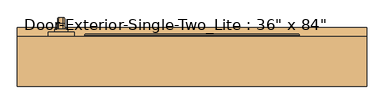
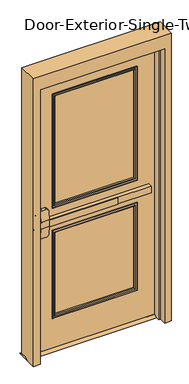
"""IFC4 building model written with IfcOpenShell, lengths in millimetres: door geometry."""

from ifc_helpers import new_model, si_unit, point, frame, frame_2d, origin, place, context, project, spatial, polyline, circle_curve, ellipse_curve, trimmed, segment, composite_curve, outline, extrude, faceted_brep, source, transform, mapped, element, save
from ifc_brep_helpers import plane_surface, cylinder_surface, revolved_surface, advanced_brep


def door_ea45fa4a(model_context):
    return source(origin(), model_context, "Body", "SolidModel", [
        extrude(outline(polyline([(61.9125, 12.7), (106.3625, 12.7), (131.7625, 0.0), (36.5125, 0.0), (61.9125, 12.7)])), frame((-508.0, 0.0, 0.0), z_axis=(1.0, 0.0, 0.0), x_axis=(0.0, 1.0, 0.0)), (0.0, 0.0, 1.0), 1016.0),
        extrude(outline(polyline([(150.2833333, 23.8125), (-349.25, 23.8125), (-349.25, 30.1625), (150.2833333, 30.1625), (150.2833333, 23.8125)])), frame((0.0, 0.0, 990.6), z_axis=(0.0, 0.0, 1.0), x_axis=(1.0, 0.0, 0.0)), (0.0, 0.0, 1.0), 50.8),
        advanced_brep(
        [(-412.75, 30.1625, 1041.4), (-412.75, 30.1625, 990.6), (-349.25, 30.1625, 990.6), (400.05, 30.1625, 990.6), (400.05, 30.1625, 1041.4), (-349.25, 30.1625, 1041.4), (400.05, 61.9125, 1041.4), (400.05, 61.9125, 990.6), (-349.25, 61.9125, 990.6), (-349.25, 61.9125, 927.1), (-368.3, 61.9125, 908.05), (-393.7, 61.9125, 908.05), (-412.75, 61.9125, 927.1), (-412.75, 61.9125, 1104.9), (-393.7, 61.9125, 1123.95), (-368.3, 61.9125, 1123.95), (-349.25, 61.9125, 1104.9), (-349.25, 61.9125, 1041.4), (-349.25, 33.3377467, 1041.4), (-412.75, 33.3377467, 1041.4), (-412.75, 38.3479269, 1104.9), (-412.75, 38.3479269, 927.1), (-412.75, 33.3377467, 990.6), (-349.25, 33.3377467, 990.6), (-349.25, 38.3479269, 927.1), (-349.25, 38.3479269, 1104.9), (-393.7, 39.850981, 1123.95), (-368.3, 39.850981, 1123.95), (-368.3, 39.850981, 908.05), (-393.7, 39.850981, 908.05)],
        [
            (0, 1),
            (1, 2),
            (2, 3),
            (3, 4),
            (4, 5),
            (5, 0),
            (6, 7),
            (7, 8),
            (8, 9),
            (9, 10, circle_curve(frame((-368.3, 61.9125, 927.1), z_axis=(0.0, 1.0, 0.0), x_axis=(1.0, 0.0, 0.0)), 19.05)),
            (10, 11),
            (11, 12, circle_curve(frame((-393.7, 61.9125, 927.1), z_axis=(0.0, 1.0, 0.0), x_axis=(1.0, 0.0, 0.0)), 19.05)),
            (12, 13),
            (13, 14, circle_curve(frame((-393.7, 61.9125, 1104.9), z_axis=(0.0, 1.0, 0.0), x_axis=(1.0, 0.0, 0.0)), 19.05)),
            (14, 15),
            (15, 16, circle_curve(frame((-368.3, 61.9125, 1104.9), z_axis=(0.0, 1.0, 0.0), x_axis=(1.0, 0.0, 0.0)), 19.05)),
            (16, 17),
            (17, 6),
            (4, 6),
            (17, 18),
            (18, 19),
            (19, 0),
            (19, 20),
            (20, 13),
            (12, 21),
            (21, 22),
            (22, 1),
            (7, 3),
            (22, 23),
            (23, 8),
            (23, 24),
            (24, 9),
            (16, 25),
            (25, 18),
            (14, 26),
            (26, 27),
            (27, 15),
            (10, 28),
            (28, 29),
            (29, 11),
            (24, 28, ellipse_curve(frame((-368.3, 38.3479269, 927.1), z_axis=(0.0, 0.9969018152893365, 0.07865602756830282), x_axis=(0.0, -0.07865602756830208, 0.9969018152893365)), 19.1092038, 19.05)),
            (27, 25, ellipse_curve(frame((-368.3, 38.3479269, 1104.9), z_axis=(0.0, 0.9969018152893376, -0.07865602756828934), x_axis=(0.0, -0.078656027568288, -0.9969018152893377)), 19.1092038, 19.05)),
            (20, 26, ellipse_curve(frame((-393.7, 38.3479269, 1104.9), z_axis=(0.0, 0.9969018152893376, -0.07865602756828934), x_axis=(0.0, -0.078656027568288, -0.9969018152893377)), 19.1092038, 19.05)),
            (29, 21, ellipse_curve(frame((-393.7, 38.3479269, 927.1), z_axis=(0.0, 0.9969018152893365, 0.07865602756830282), x_axis=(0.0, -0.07865602756830208, 0.9969018152893365)), 19.1092038, 19.05)),
        ],
        [
            plane_surface(frame((-412.75, 30.1625, 1041.4), z_axis=(0.0, -1.0, 0.0), x_axis=(-1.0, 0.0, 0.0))),
            plane_surface(frame((-412.75, 61.9125, 1041.4), z_axis=(0.0, 1.0, 0.0), x_axis=(1.0, 0.0, 0.0))),
            plane_surface(frame((400.05, 30.1625, 1041.4), z_axis=(0.0, 0.0, 1.0), x_axis=(0.0, 1.0, 0.0))),
            plane_surface(frame((-412.75, 30.1625, 1041.4), z_axis=(-1.0, 0.0, 0.0), x_axis=(0.0, 1.0, 0.0))),
            plane_surface(frame((-412.75, 30.1625, 990.6), z_axis=(0.0, 0.0, -1.0), x_axis=(0.0, 1.0, 0.0))),
            plane_surface(frame((400.05, 30.1625, 990.6), z_axis=(1.0, 0.0, 0.0), x_axis=(0.0, 1.0, 0.0))),
            plane_surface(frame((-349.25, 33.3377467, 927.1), z_axis=(1.0, 0.0, 0.0), x_axis=(0.0, 1.0, 0.0))),
            plane_surface(frame((-368.3, 33.3377467, 1123.95), z_axis=(0.0, 0.0, 1.0), x_axis=(0.0, 1.0, 0.0))),
            plane_surface(frame((-393.7, 33.3377467, 908.05), z_axis=(0.0, 0.0, -1.0), x_axis=(0.0, 1.0, 0.0))),
            cylinder_surface(frame((-368.3, 61.9125, 927.1), z_axis=(0.0, -1.0, 0.0), x_axis=(1.0, 0.0, 0.0)), 19.05),
            cylinder_surface(frame((-368.3, 61.9125, 1104.9), z_axis=(0.0, -1.0, 0.0), x_axis=(1.0, 0.0, 0.0)), 19.05),
            cylinder_surface(frame((-393.7, 61.9125, 1104.9), z_axis=(0.0, -1.0, 0.0), x_axis=(1.0, 0.0, 0.0)), 19.05),
            cylinder_surface(frame((-393.7, 61.9125, 927.1), z_axis=(0.0, -1.0, 0.0), x_axis=(1.0, 0.0, 0.0)), 19.05),
            plane_surface(frame((-349.25, 33.3377467, 1041.4), z_axis=(0.0, -0.9969018152893376, 0.07865602756828934), x_axis=(-1.0, 0.0, 0.0))),
            plane_surface(frame((-349.25, 39.850981, 908.05), z_axis=(0.0, -0.9969018152893365, -0.07865602756830282), x_axis=(-1.0, 0.0, 0.0))),
        ],
        [
            (0, [[1, 2, 3, 4, 5, 6]]),
            (1, [[7, 8, 9, 10, 11, 12, 13, 14, 15, 16, 17, 18]]),
            (2, [[19, -18, 20, 21, 22, -6, -5]]),
            (3, [[-1, -22, 23, 24, -13, 25, 26, 27]]),
            (4, [[28, -3, -2, -27, 29, 30, -8]]),
            (5, [[-4, -28, -7, -19]]),
            (6, [[-9, -30, 31, 32]]),
            (6, [[-17, 33, 34, -20]]),
            (7, [[-15, 35, 36, 37]]),
            (8, [[-11, 38, 39, 40]]),
            (9, [[-10, -32, 41, -38]]),
            (10, [[-16, -37, 42, -33]]),
            (11, [[-14, -24, 43, -35]]),
            (12, [[-12, -40, 44, -25]]),
            (13, [[-21, -34, -42, -36, -43, -23]]),
            (14, [[-26, -44, -39, -41, -31, -29]]),
        ],
    ),
        advanced_brep(
        [(-391.0, 119.0625, 1017.190625), (-391.0, 119.0625, 1014.809375), (-387.428125, 119.0625, 1011.2375), (-374.5715406, 119.0625, 1011.2375), (-371.0, 119.0625, 1014.8090406), (-371.0, 119.0625, 1017.190625), (-374.571875, 119.0625, 1020.7625), (-387.428125, 119.0625, 1020.7625), (-391.0, 119.0625, 887.809375), (-387.428125, 119.0625, 884.2375), (-374.571875, 119.0625, 884.2375), (-371.0, 119.0625, 887.809375), (-371.0, 119.0625, 890.1909594), (-374.5715406, 119.0625, 893.7625), (-387.428125, 119.0625, 893.7625), (-391.0, 119.0625, 890.190625), (-391.0, 144.4625, 1017.190625), (-391.0, 158.353125, 1003.3), (-391.0, 158.353125, 901.7), (-391.0, 144.4625, 887.809375), (-391.0, 144.4625, 890.190625), (-391.0, 155.971875, 901.7), (-391.0, 155.971875, 1003.3), (-391.0, 144.4625, 1014.809375), (-387.428125, 144.4625, 1011.2375), (-374.5715406, 144.4625, 1011.2375), (-371.0, 144.4625, 1014.8090406), (-371.0, 155.9715406, 1003.3), (-371.0, 155.9715406, 901.7), (-371.0, 144.4625, 890.1909594), (-371.0, 144.4625, 887.809375), (-371.0, 158.353125, 901.7), (-371.0, 158.353125, 1003.3), (-371.0, 144.4625, 1017.190625), (-374.571875, 144.4625, 1020.7625), (-387.428125, 144.4625, 1020.7625), (-387.428125, 152.4, 1003.3), (-374.5715406, 152.4, 1003.3), (-374.571875, 161.925, 1003.3), (-387.428125, 161.925, 1003.3), (-387.428125, 152.4, 901.7), (-374.5715406, 152.4, 901.7), (-374.571875, 161.925, 901.7), (-387.428125, 161.925, 901.7), (-387.428125, 144.4625, 893.7625), (-374.5715406, 144.4625, 893.7625), (-374.571875, 144.4625, 884.2375), (-387.428125, 144.4625, 884.2375)],
        [
            (0, 1),
            (1, 2, circle_curve(frame((-387.428125, 119.0625, 1014.809375), z_axis=(0.0, -1.0, 0.0), x_axis=(0.0, 0.0, 1.0)), 3.571875)),
            (2, 3),
            (3, 4, circle_curve(frame((-374.5715406, 119.0625, 1014.8090406), z_axis=(0.0, -1.0, 0.0), x_axis=(0.0, 0.0, 1.0)), 3.5715406)),
            (4, 5),
            (5, 6, circle_curve(frame((-374.571875, 119.0625, 1017.190625), z_axis=(0.0, -1.0, 0.0), x_axis=(0.0, 0.0, 1.0)), 3.571875)),
            (6, 7),
            (7, 0, circle_curve(frame((-387.428125, 119.0625, 1017.190625), z_axis=(0.0, -1.0, 0.0), x_axis=(0.0, 0.0, 1.0)), 3.571875)),
            (8, 9, circle_curve(frame((-387.428125, 119.0625, 887.809375), z_axis=(0.0, -1.0, 0.0), x_axis=(0.0, 0.0, -1.0)), 3.571875)),
            (9, 10),
            (10, 11, circle_curve(frame((-374.571875, 119.0625, 887.809375), z_axis=(0.0, -1.0, 0.0), x_axis=(0.0, 0.0, -1.0)), 3.571875)),
            (11, 12),
            (12, 13, circle_curve(frame((-374.5715406, 119.0625, 890.1909594), z_axis=(0.0, -1.0, 0.0), x_axis=(0.0, 0.0, -1.0)), 3.5715406)),
            (13, 14),
            (14, 15, circle_curve(frame((-387.428125, 119.0625, 890.190625), z_axis=(0.0, -1.0, 0.0), x_axis=(0.0, 0.0, -1.0)), 3.571875)),
            (15, 8),
            (0, 16),
            (16, 17, circle_curve(frame((-391.0, 144.4625, 1003.3), z_axis=(-1.0, 0.0, 0.0), x_axis=(0.0, 0.0, 1.0)), 13.890625)),
            (17, 18),
            (18, 19, circle_curve(frame((-391.0, 144.4625, 901.7), z_axis=(-1.0, 0.0, 0.0), x_axis=(0.0, 1.0, 0.0)), 13.890625)),
            (19, 8),
            (15, 20),
            (20, 21, circle_curve(frame((-391.0, 144.4625, 901.7), z_axis=(1.0, 0.0, 0.0), x_axis=(0.0, 1.0, 0.0)), 11.509375)),
            (21, 22),
            (22, 23, circle_curve(frame((-391.0, 144.4625, 1003.3), z_axis=(1.0, 0.0, 0.0), x_axis=(0.0, 0.0, 1.0)), 11.509375)),
            (23, 1),
            (23, 24, circle_curve(frame((-387.428125, 144.4625, 1014.809375), z_axis=(0.0, -1.0, 0.0), x_axis=(0.0, 0.0, 1.0)), 3.571875)),
            (24, 2),
            (24, 25),
            (25, 3),
            (25, 26, circle_curve(frame((-374.5715406, 144.4625, 1014.8090406), z_axis=(0.0, -1.0, 0.0), x_axis=(0.0, 0.0, 1.0)), 3.5715406)),
            (26, 4),
            (26, 27, circle_curve(frame((-371.0, 144.4625, 1003.3), z_axis=(-1.0, 0.0, 0.0), x_axis=(0.0, 0.0, 1.0)), 11.5090406)),
            (27, 28),
            (28, 29, circle_curve(frame((-371.0, 144.4625, 901.7), z_axis=(-1.0, 0.0, 0.0), x_axis=(0.0, 1.0, 0.0)), 11.5090406)),
            (29, 12),
            (11, 30),
            (30, 31, circle_curve(frame((-371.0, 144.4625, 901.7), z_axis=(1.0, 0.0, 0.0), x_axis=(0.0, 1.0, 0.0)), 13.890625)),
            (31, 32),
            (32, 33, circle_curve(frame((-371.0, 144.4625, 1003.3), z_axis=(1.0, 0.0, 0.0), x_axis=(0.0, 0.0, 1.0)), 13.890625)),
            (33, 5),
            (33, 34, circle_curve(frame((-374.571875, 144.4625, 1017.190625), z_axis=(0.0, -1.0, 0.0), x_axis=(0.0, 0.0, 1.0)), 3.571875)),
            (34, 6),
            (34, 35),
            (35, 7),
            (35, 16, circle_curve(frame((-387.428125, 144.4625, 1017.190625), z_axis=(0.0, -1.0, 0.0), x_axis=(0.0, 0.0, 1.0)), 3.571875)),
            (36, 24, circle_curve(frame((-387.428125, 144.4625, 1003.3), z_axis=(1.0, 0.0, 0.0), x_axis=(0.0, 0.0, 1.0)), 7.9375)),
            (22, 36, circle_curve(frame((-387.428125, 155.971875, 1003.3), z_axis=(0.0, 0.0, 1.0), x_axis=(0.0, 1.0, 0.0)), 3.571875)),
            (37, 25, circle_curve(frame((-374.5715406, 144.4625, 1003.3), z_axis=(1.0, 0.0, 0.0), x_axis=(0.0, 0.0, 1.0)), 7.9375)),
            (36, 37),
            (37, 27, circle_curve(frame((-374.5715406, 155.9715406, 1003.3), z_axis=(0.0, 0.0, 1.0), x_axis=(0.0, 1.0, 0.0)), 3.5715406)),
            (38, 34, circle_curve(frame((-374.571875, 144.4625, 1003.3), z_axis=(1.0, 0.0, 0.0), x_axis=(0.0, 0.0, 1.0)), 17.4625)),
            (32, 38, circle_curve(frame((-374.571875, 158.353125, 1003.3), z_axis=(0.0, 0.0, 1.0), x_axis=(0.0, 1.0, 0.0)), 3.571875)),
            (39, 35, circle_curve(frame((-387.428125, 144.4625, 1003.3), z_axis=(1.0, 0.0, 0.0), x_axis=(0.0, 0.0, 1.0)), 17.4625)),
            (38, 39),
            (39, 17, circle_curve(frame((-387.428125, 158.353125, 1003.3), z_axis=(0.0, 0.0, 1.0), x_axis=(0.0, 1.0, 0.0)), 3.571875)),
            (21, 40, circle_curve(frame((-387.428125, 155.971875, 901.7), z_axis=(0.0, 0.0, 1.0), x_axis=(0.0, 1.0, 0.0)), 3.571875)),
            (40, 36),
            (40, 41),
            (41, 37),
            (41, 28, circle_curve(frame((-374.5715406, 155.9715406, 901.7), z_axis=(0.0, 0.0, 1.0), x_axis=(0.0, 1.0, 0.0)), 3.5715406)),
            (31, 42, circle_curve(frame((-374.571875, 158.353125, 901.7), z_axis=(0.0, 0.0, 1.0), x_axis=(0.0, 1.0, 0.0)), 3.571875)),
            (42, 38),
            (42, 43),
            (43, 39),
            (43, 18, circle_curve(frame((-387.428125, 158.353125, 901.7), z_axis=(0.0, 0.0, 1.0), x_axis=(0.0, 1.0, 0.0)), 3.571875)),
            (44, 40, circle_curve(frame((-387.428125, 144.4625, 901.7), z_axis=(1.0, 0.0, 0.0), x_axis=(0.0, 1.0, 0.0)), 7.9375)),
            (20, 44, circle_curve(frame((-387.428125, 144.4625, 890.190625), z_axis=(0.0, 1.0, 0.0), x_axis=(0.0, 0.0, -1.0)), 3.571875)),
            (45, 41, circle_curve(frame((-374.5715406, 144.4625, 901.7), z_axis=(1.0, 0.0, 0.0), x_axis=(0.0, 1.0, 0.0)), 7.9375)),
            (44, 45),
            (45, 29, circle_curve(frame((-374.5715406, 144.4625, 890.1909594), z_axis=(0.0, 1.0, 0.0), x_axis=(0.0, 0.0, -1.0)), 3.5715406)),
            (46, 42, circle_curve(frame((-374.571875, 144.4625, 901.7), z_axis=(1.0, 0.0, 0.0), x_axis=(0.0, 1.0, 0.0)), 17.4625)),
            (30, 46, circle_curve(frame((-374.571875, 144.4625, 887.809375), z_axis=(0.0, 1.0, 0.0), x_axis=(0.0, 0.0, -1.0)), 3.571875)),
            (47, 43, circle_curve(frame((-387.428125, 144.4625, 901.7), z_axis=(1.0, 0.0, 0.0), x_axis=(0.0, 1.0, 0.0)), 17.4625)),
            (46, 47),
            (47, 19, circle_curve(frame((-387.428125, 144.4625, 887.809375), z_axis=(0.0, 1.0, 0.0), x_axis=(0.0, 0.0, -1.0)), 3.571875)),
            (14, 44),
            (13, 45),
            (10, 46),
            (9, 47),
        ],
        [
            plane_surface(frame((-381.0, 119.0625, 1016.0), z_axis=(0.0, -1.0, 0.0), x_axis=(1.0, 0.0, 0.0))),
            plane_surface(frame((-381.0, 119.0625, 889.0), z_axis=(0.0, -1.0, 0.0), x_axis=(1.0, 0.0, 0.0))),
            plane_surface(frame((-391.0, 119.0625, 1017.190625), z_axis=(-1.0, 0.0, 0.0), x_axis=(0.0, 1.0, 0.0))),
            cylinder_surface(frame((-387.428125, 119.0625, 1014.809375), z_axis=(0.0, -1.0, 0.0), x_axis=(0.0, 0.0, 1.0)), 3.571875),
            plane_surface(frame((-387.428125, 119.0625, 1011.2375), z_axis=(0.0, 0.0, -1.0), x_axis=(0.0, 1.0, 0.0))),
            cylinder_surface(frame((-374.5715406, 119.0625, 1014.8090406), z_axis=(0.0, -1.0, 0.0), x_axis=(0.0, 0.0, 1.0)), 3.5715406),
            plane_surface(frame((-371.0, 119.0625, 1014.8090406), z_axis=(1.0, 0.0, 0.0), x_axis=(0.0, 1.0, 0.0))),
            cylinder_surface(frame((-374.571875, 119.0625, 1017.190625), z_axis=(0.0, -1.0, 0.0), x_axis=(0.0, 0.0, 1.0)), 3.571875),
            plane_surface(frame((-374.571875, 119.0625, 1020.7625), z_axis=(0.0, 0.0, 1.0), x_axis=(0.0, 1.0, 0.0))),
            cylinder_surface(frame((-387.428125, 119.0625, 1017.190625), z_axis=(0.0, -1.0, 0.0), x_axis=(0.0, 0.0, 1.0)), 3.571875),
            revolved_surface(trimmed(ellipse_curve(frame((-387.428125, 144.4625, 1014.809375), z_axis=(0.0, -1.0, 0.0), x_axis=(0.0, 0.0, 1.0)), 3.571875, 3.571875), [point((-391.0, 144.4625, 1014.809375))], [point((-387.428125, 144.4625, 1011.2375))], True, "CARTESIAN"), (-381.0, 144.4625, 1003.3), (-1.0, 0.0, 0.0)),
            revolved_surface(polyline([(-387.428125, 144.4625, 1011.2375), (-374.5715406, 144.4625, 1011.2375)]), (-381.0, 144.4625, 1003.3), (-1.0, 0.0, 0.0)),
            revolved_surface(trimmed(ellipse_curve(frame((-374.5715406, 144.4625, 1014.8090406), z_axis=(0.0, -1.0, 0.0), x_axis=(0.0, 0.0, 1.0)), 3.5715406, 3.5715406), [point((-374.5715406, 144.4625, 1011.2375))], [point((-371.0, 144.4625, 1014.8090406))], True, "CARTESIAN"), (-381.0, 144.4625, 1003.3), (-1.0, 0.0, 0.0)),
            revolved_surface(trimmed(ellipse_curve(frame((-374.571875, 144.4625, 1017.190625), z_axis=(0.0, -1.0, 0.0), x_axis=(0.0, 0.0, 1.0)), 3.571875, 3.571875), [point((-371.0, 144.4625, 1017.190625))], [point((-374.571875, 144.4625, 1020.7625))], True, "CARTESIAN"), (-381.0, 144.4625, 1003.3), (-1.0, 0.0, 0.0)),
            cylinder_surface(frame((-381.0, 144.4625, 1003.3), z_axis=(-1.0, 0.0, 0.0), x_axis=(0.0, 0.0, 1.0)), 17.4625),
            revolved_surface(trimmed(ellipse_curve(frame((-387.428125, 144.4625, 1017.190625), z_axis=(0.0, -1.0, 0.0), x_axis=(0.0, 0.0, 1.0)), 3.571875, 3.571875), [point((-387.428125, 144.4625, 1020.7625))], [point((-391.0, 144.4625, 1017.190625))], True, "CARTESIAN"), (-381.0, 144.4625, 1003.3), (-1.0, 0.0, 0.0)),
            cylinder_surface(frame((-387.428125, 155.971875, 1003.3), z_axis=(0.0, 0.0, 1.0), x_axis=(0.0, 1.0, 0.0)), 3.571875),
            plane_surface(frame((-387.428125, 152.4, 1003.3), z_axis=(0.0, -1.0, 0.0), x_axis=(0.0, 0.0, -1.0))),
            cylinder_surface(frame((-374.5715406, 155.9715406, 1003.3), z_axis=(0.0, 0.0, 1.0), x_axis=(0.0, 1.0, 0.0)), 3.5715406),
            cylinder_surface(frame((-374.571875, 158.353125, 1003.3), z_axis=(0.0, 0.0, 1.0), x_axis=(0.0, 1.0, 0.0)), 3.571875),
            plane_surface(frame((-374.571875, 161.925, 1003.3), z_axis=(0.0, 1.0, 0.0), x_axis=(0.0, 0.0, -1.0))),
            cylinder_surface(frame((-387.428125, 158.353125, 1003.3), z_axis=(0.0, 0.0, 1.0), x_axis=(0.0, 1.0, 0.0)), 3.571875),
            revolved_surface(trimmed(ellipse_curve(frame((-387.428125, 155.971875, 901.7), z_axis=(0.0, 0.0, 1.0), x_axis=(0.0, 1.0, 0.0)), 3.571875, 3.571875), [point((-391.0, 155.971875, 901.7))], [point((-387.428125, 152.4, 901.7))], True, "CARTESIAN"), (-381.0, 144.4625, 901.7), (-1.0, 0.0, 0.0)),
            revolved_surface(polyline([(-387.428125, 152.4, 901.7), (-374.5715406, 152.4, 901.7)]), (-381.0, 144.4625, 901.7), (-1.0, 0.0, 0.0)),
            revolved_surface(trimmed(ellipse_curve(frame((-374.5715406, 155.9715406, 901.7), z_axis=(0.0, 0.0, 1.0), x_axis=(0.0, 1.0, 0.0)), 3.5715406, 3.5715406), [point((-374.5715406, 152.4, 901.7))], [point((-371.0, 155.9715406, 901.7))], True, "CARTESIAN"), (-381.0, 144.4625, 901.7), (-1.0, 0.0, 0.0)),
            revolved_surface(trimmed(ellipse_curve(frame((-374.571875, 158.353125, 901.7), z_axis=(0.0, 0.0, 1.0), x_axis=(0.0, 1.0, 0.0)), 3.571875, 3.571875), [point((-371.0, 158.353125, 901.7))], [point((-374.571875, 161.925, 901.7))], True, "CARTESIAN"), (-381.0, 144.4625, 901.7), (-1.0, 0.0, 0.0)),
            cylinder_surface(frame((-381.0, 144.4625, 901.7), z_axis=(-1.0, 0.0, 0.0), x_axis=(0.0, 1.0, 0.0)), 17.4625),
            revolved_surface(trimmed(ellipse_curve(frame((-387.428125, 158.353125, 901.7), z_axis=(0.0, 0.0, 1.0), x_axis=(0.0, 1.0, 0.0)), 3.571875, 3.571875), [point((-387.428125, 161.925, 901.7))], [point((-391.0, 158.353125, 901.7))], True, "CARTESIAN"), (-381.0, 144.4625, 901.7), (-1.0, 0.0, 0.0)),
            cylinder_surface(frame((-387.428125, 144.4625, 890.190625), z_axis=(0.0, 1.0, 0.0), x_axis=(0.0, 0.0, -1.0)), 3.571875),
            plane_surface(frame((-387.428125, 144.4625, 893.7625), z_axis=(0.0, 0.0, 1.0), x_axis=(0.0, -1.0, 0.0))),
            cylinder_surface(frame((-374.5715406, 144.4625, 890.1909594), z_axis=(0.0, 1.0, 0.0), x_axis=(0.0, 0.0, -1.0)), 3.5715406),
            cylinder_surface(frame((-374.571875, 144.4625, 887.809375), z_axis=(0.0, 1.0, 0.0), x_axis=(0.0, 0.0, -1.0)), 3.571875),
            plane_surface(frame((-374.571875, 144.4625, 884.2375), z_axis=(0.0, 0.0, -1.0), x_axis=(0.0, -1.0, 0.0))),
            cylinder_surface(frame((-387.428125, 144.4625, 887.809375), z_axis=(0.0, 1.0, 0.0), x_axis=(0.0, 0.0, -1.0)), 3.571875),
        ],
        [
            (0, [[1, 2, 3, 4, 5, 6, 7, 8]]),
            (1, [[9, 10, 11, 12, 13, 14, 15, 16]]),
            (2, [[-1, 17, 18, 19, 20, 21, -16, 22, 23, 24, 25, 26]]),
            (3, [[-2, -26, 27, 28]]),
            (4, [[-3, -28, 29, 30]]),
            (5, [[-4, -30, 31, 32]]),
            (6, [[-5, -32, 33, 34, 35, 36, -12, 37, 38, 39, 40, 41]]),
            (7, [[-6, -41, 42, 43]]),
            (8, [[-7, -43, 44, 45]]),
            (9, [[-8, -45, 46, -17]]),
            (10, [[47, -27, -25, 48]]),
            (11, [[49, -29, -47, 50]]),
            (12, [[-33, -31, -49, 51]]),
            (13, [[52, -42, -40, 53]]),
            (14, [[54, -44, -52, 55]]),
            (15, [[-18, -46, -54, 56]]),
            (16, [[-48, -24, 57, 58]]),
            (17, [[-50, -58, 59, 60]]),
            (18, [[-51, -60, 61, -34]]),
            (19, [[-53, -39, 62, 63]]),
            (20, [[-55, -63, 64, 65]]),
            (21, [[-56, -65, 66, -19]]),
            (22, [[67, -57, -23, 68]]),
            (23, [[69, -59, -67, 70]]),
            (24, [[-35, -61, -69, 71]]),
            (25, [[72, -62, -38, 73]]),
            (26, [[74, -64, -72, 75]]),
            (27, [[-20, -66, -74, 76]]),
            (28, [[-68, -22, -15, 77]]),
            (29, [[-70, -77, -14, 78]]),
            (30, [[-71, -78, -13, -36]]),
            (31, [[-73, -37, -11, 79]]),
            (32, [[-75, -79, -10, 80]]),
            (33, [[-76, -80, -9, -21]]),
        ],
    ),
        extrude(outline(composite_curve([segment(trimmed(circle_curve(frame_2d((1117.6, -381.0)), 19.0), [point((1117.6, -400.0))], [point((1117.6, -362.0))], False, "CARTESIAN"), True, "CONTINUOUS"), segment(trimmed(circle_curve(frame_2d((1117.6, -381.0)), 19.0), [point((1117.6, -362.0))], [point((1117.6, -400.0))], False, "CARTESIAN"), True, "CONTINUOUS")], self_intersect=False)), frame((0.0, 119.0625, 0.0), z_axis=(0.0, 1.0, 0.0), x_axis=(0.0, 0.0, 1.0)), (0.0, 0.0, 1.0), 8.73125),
        extrude(outline(composite_curve([segment(trimmed(circle_curve(frame_2d((1113.0338574, -381.0)), 89.3016225), [point((1193.8, -342.9))], [point((1193.8, -419.1))], False, "CARTESIAN"), True, "CONTINUOUS"), segment(polyline([(1193.8, -419.1), (838.2, -419.1)]), True, "CONTINUOUS"), segment(trimmed(circle_curve(frame_2d((918.9661426, -381.0)), 89.3016225), [point((838.2, -419.1))], [point((838.2, -342.9))], False, "CARTESIAN"), True, "CONTINUOUS"), segment(polyline([(838.2, -342.9), (1193.8, -342.9)]), True, "CONTINUOUS")], self_intersect=False)), frame((0.0, 106.3625, 0.0), z_axis=(0.0, 1.0, 0.0), x_axis=(0.0, 0.0, 1.0)), (0.0, 0.0, 1.0), 12.7),
        faceted_brep([(457.2, 57.15, 0.0), (457.2, 106.3625, 0.0), (508.0, 106.3625, 0.0), (508.0, -39.6875, 0.0), (457.2, -39.6875, 0.0), (457.2, 9.525, 0.0), (441.325, 9.525, 0.0), (441.325, 57.15, 0.0), (457.2, 57.15, 2133.6), (457.2, 106.3625, 2133.6), (-457.2, 106.3625, 2133.6), (-457.2, 106.3625, 0.0), (-508.0, 106.3625, 0.0), (-508.0, 106.3625, 2235.2), (508.0, 106.3625, 2235.2), (508.0, -39.6875, 2235.2), (-508.0, -39.6875, 2235.2), (-508.0, -39.6875, 0.0), (-457.2, -39.6875, 0.0), (-457.2, -39.6875, 2133.6), (457.2, -39.6875, 2133.6), (457.2, 9.525, 2133.6), (-457.2, 9.525, 2133.6), (-457.2, 9.525, 0.0), (-441.325, 9.525, 0.0), (-441.325, 9.525, 2117.725), (441.325, 9.525, 2117.725), (441.325, 57.15, 2117.725), (-441.325, 57.15, 2117.725), (-441.325, 57.15, 0.0), (-457.2, 57.15, 0.0), (-457.2, 57.15, 2133.6)], [[[0, 1, 2, 3, 4, 5, 6, 7]], [[1, 0, 8, 9]], [[2, 1, 9, 10, 11, 12, 13, 14]], [[3, 2, 14, 15]], [[4, 3, 15, 16, 17, 18, 19, 20]], [[5, 4, 20, 21]], [[6, 5, 21, 22, 23, 24, 25, 26]], [[7, 6, 26, 27]], [[0, 7, 27, 28, 29, 30, 31, 8]], [[9, 8, 31, 10]], [[20, 19, 22, 21]], [[26, 25, 28, 27]], [[12, 11, 30, 29, 24, 23, 18, 17]], [[11, 10, 31, 30]], [[13, 12, 17, 16]], [[19, 18, 23, 22]], [[25, 24, 29, 28]], [[15, 14, 13, 16]]]),
        extrude(outline(polyline([(2133.6, -457.2), (12.7, -457.2), (12.7, 457.2), (2133.6, 457.2), (2133.6, -457.2)]), holes=[polyline([(1981.2, -304.8), (1981.2, 304.8), (1111.25, 304.8), (1111.25, -304.8), (1981.2, -304.8)]), polyline([(920.75, -304.8), (920.75, 304.8), (254.0, 304.8), (254.0, -304.8), (920.75, -304.8)])]), frame((0.0, 61.9125, 0.0), z_axis=(0.0, 1.0, 0.0), x_axis=(0.0, 0.0, 1.0)), (0.0, 0.0, 1.0), 44.45),
        extrude(outline(polyline([(304.8, 74.6125), (-304.8, 74.6125), (-304.8, 93.6625), (304.8, 93.6625), (304.8, 74.6125)])), frame((0.0, 0.0, 1111.25), z_axis=(0.0, 0.0, 1.0), x_axis=(1.0, 0.0, 0.0)), (0.0, 0.0, 1.0), 869.95),
        extrude(outline(polyline([(304.8, 74.6125), (-304.8, 74.6125), (-304.8, 93.6625), (304.8, 93.6625), (304.8, 74.6125)])), frame((0.0, 0.0, 254.0), z_axis=(0.0, 0.0, 1.0), x_axis=(1.0, 0.0, 0.0)), (0.0, 0.0, 1.0), 666.75),
        advanced_brep(
        [(304.8, 74.6125, 920.75), (304.8, 61.9125, 920.75), (304.8, 61.9125, 254.0), (304.8, 74.6125, 254.0), (292.8, 60.9125, 908.75), (292.8, 74.6125, 908.75), (292.8, 74.6125, 266.0), (292.8, 60.9125, 266.0), (297.8, 55.9125, 913.75), (297.8, 55.9125, 261.0), (312.8, 57.9125, 928.75), (310.8, 55.9125, 926.75), (310.8, 55.9125, 248.0), (312.8, 57.9125, 246.0), (312.8, 61.9125, 928.75), (312.8, 61.9125, 246.0), (-304.8, 61.9125, 254.0), (-304.8, 74.6125, 254.0), (-292.8, 74.6125, 266.0), (-292.8, 60.9125, 266.0), (-297.8, 55.9125, 261.0), (-310.8, 55.9125, 248.0), (-312.8, 57.9125, 246.0), (-312.8, 61.9125, 246.0), (-304.8, 61.9125, 920.75), (-304.8, 74.6125, 920.75), (-292.8, 74.6125, 908.75), (-292.8, 60.9125, 908.75), (-297.8, 55.9125, 913.75), (-310.8, 55.9125, 926.75), (-312.8, 57.9125, 928.75), (-312.8, 61.9125, 928.75)],
        [
            (0, 1),
            (1, 2),
            (2, 3),
            (3, 0),
            (4, 5),
            (5, 6),
            (6, 7),
            (7, 4),
            (8, 4, ellipse_curve(frame((297.8, 60.9125, 913.75), z_axis=(0.7071067811865475, 0.0, -0.7071067811865475), x_axis=(0.7071067811865474, 0.0, 0.7071067811865476)), 7.0710678, 5.0)),
            (7, 9, ellipse_curve(frame((297.8, 60.9125, 261.0), z_axis=(0.7071067811865475, 0.0, 0.7071067811865475), x_axis=(-0.7071067811865474, 0.0, 0.7071067811865476)), 7.0710678, 5.0)),
            (9, 8),
            (10, 11, ellipse_curve(frame((310.8, 57.9125, 926.75), z_axis=(0.7071067811865475, 0.0, -0.7071067811865475), x_axis=(0.7071067811865474, 0.0, 0.7071067811865476)), 2.8284271, 2.0)),
            (11, 12),
            (12, 13, ellipse_curve(frame((310.8, 57.9125, 248.0), z_axis=(0.7071067811865475, 0.0, 0.7071067811865475), x_axis=(-0.7071067811865474, 0.0, 0.7071067811865476)), 2.8284271, 2.0)),
            (13, 10),
            (14, 10),
            (13, 15),
            (15, 14),
            (2, 16),
            (16, 17),
            (17, 3),
            (6, 18),
            (18, 19),
            (19, 7),
            (19, 20, ellipse_curve(frame((-297.8, 60.9125, 261.0), z_axis=(0.7071067811865475, 0.0, -0.7071067811865475), x_axis=(0.7071067811865476, 0.0, 0.7071067811865474)), 7.0710678, 5.0)),
            (20, 9),
            (12, 21),
            (21, 22, ellipse_curve(frame((-310.8, 57.9125, 248.0), z_axis=(0.7071067811865475, 0.0, -0.7071067811865475), x_axis=(0.7071067811865476, 0.0, 0.7071067811865474)), 2.8284271, 2.0)),
            (22, 13),
            (22, 23),
            (23, 15),
            (16, 24),
            (24, 25),
            (25, 17),
            (18, 26),
            (26, 27),
            (27, 19),
            (27, 28, ellipse_curve(frame((-297.8, 60.9125, 913.75), z_axis=(-0.7071067811865475, 0.0, -0.7071067811865475), x_axis=(0.7071067811865474, 0.0, -0.7071067811865476)), 7.0710678, 5.0)),
            (28, 20),
            (21, 29),
            (29, 30, ellipse_curve(frame((-310.8, 57.9125, 926.75), z_axis=(-0.7071067811865475, 0.0, -0.7071067811865475), x_axis=(0.7071067811865474, 0.0, -0.7071067811865476)), 2.8284271, 2.0)),
            (30, 22),
            (30, 31),
            (31, 23),
            (31, 14),
            (1, 24),
            (0, 25),
            (5, 26),
            (4, 27),
            (8, 28),
            (11, 29),
            (10, 30),
        ],
        [
            plane_surface(frame((304.8, 61.9125, 920.75), z_axis=(1.0, 0.0, 0.0), x_axis=(0.0, 0.0, -1.0))),
            plane_surface(frame((292.8, 74.6125, 908.75), z_axis=(-1.0, 0.0, 0.0), x_axis=(0.0, 0.0, -1.0))),
            cylinder_surface(frame((297.8, 60.9125, 920.75), z_axis=(0.0, 0.0, 1.0), x_axis=(1.0, 0.0, 0.0)), 5.0),
            cylinder_surface(frame((310.8, 57.9125, 920.75), z_axis=(0.0, 0.0, 1.0), x_axis=(1.0, 0.0, 0.0)), 2.0),
            plane_surface(frame((312.8, 57.9125, 928.75), z_axis=(1.0, 0.0, 0.0), x_axis=(0.0, 0.0, -1.0))),
            plane_surface(frame((304.8, 61.9125, 254.0), z_axis=(0.0, 0.0, -1.0), x_axis=(-1.0, 0.0, 0.0))),
            plane_surface(frame((292.8, 74.6125, 266.0), z_axis=(0.0, 0.0, 1.0), x_axis=(-1.0, 0.0, 0.0))),
            cylinder_surface(frame((304.8, 60.9125, 261.0), z_axis=(1.0, 0.0, 0.0), x_axis=(0.0, 0.0, -1.0)), 5.0),
            cylinder_surface(frame((304.8, 57.9125, 248.0), z_axis=(1.0, 0.0, 0.0), x_axis=(0.0, 0.0, -1.0)), 2.0),
            plane_surface(frame((312.8, 57.9125, 246.0), z_axis=(0.0, 0.0, -1.0), x_axis=(-1.0, 0.0, 0.0))),
            plane_surface(frame((-304.8, 61.9125, 254.0), z_axis=(-1.0, 0.0, 0.0), x_axis=(0.0, 0.0, 1.0))),
            plane_surface(frame((-292.8, 74.6125, 266.0), z_axis=(1.0, 0.0, 0.0), x_axis=(0.0, 0.0, 1.0))),
            cylinder_surface(frame((-297.8, 60.9125, 254.0), z_axis=(0.0, 0.0, -1.0), x_axis=(-1.0, 0.0, 0.0)), 5.0),
            cylinder_surface(frame((-310.8, 57.9125, 254.0), z_axis=(0.0, 0.0, -1.0), x_axis=(-1.0, 0.0, 0.0)), 2.0),
            plane_surface(frame((-312.8, 57.9125, 246.0), z_axis=(-1.0, 0.0, 0.0), x_axis=(0.0, 0.0, 1.0))),
            plane_surface(frame((-312.8, 61.9125, 928.75), z_axis=(0.0, 1.0, 0.0), x_axis=(1.0, 0.0, 0.0))),
            plane_surface(frame((-304.8, 61.9125, 920.75), z_axis=(0.0, 0.0, 1.0), x_axis=(1.0, 0.0, 0.0))),
            plane_surface(frame((-304.8, 74.6125, 920.75), z_axis=(0.0, 1.0, 0.0), x_axis=(1.0, 0.0, 0.0))),
            plane_surface(frame((-292.8, 74.6125, 908.75), z_axis=(0.0, 0.0, -1.0), x_axis=(1.0, 0.0, 0.0))),
            cylinder_surface(frame((-304.8, 60.9125, 913.75), z_axis=(-1.0, 0.0, 0.0), x_axis=(0.0, 0.0, 1.0)), 5.0),
            plane_surface(frame((-297.8, 55.9125, 913.75), z_axis=(0.0, -1.0, 0.0), x_axis=(1.0, 0.0, 0.0))),
            cylinder_surface(frame((-304.8, 57.9125, 926.75), z_axis=(-1.0, 0.0, 0.0), x_axis=(0.0, 0.0, 1.0)), 2.0),
            plane_surface(frame((-312.8, 57.9125, 928.75), z_axis=(0.0, 0.0, 1.0), x_axis=(1.0, 0.0, 0.0))),
        ],
        [
            (0, [[1, 2, 3, 4]]),
            (1, [[5, 6, 7, 8]]),
            (2, [[9, -8, 10, 11]]),
            (3, [[12, 13, 14, 15]]),
            (4, [[16, -15, 17, 18]]),
            (5, [[-3, 19, 20, 21]]),
            (6, [[-7, 22, 23, 24]]),
            (7, [[-10, -24, 25, 26]]),
            (8, [[-14, 27, 28, 29]]),
            (9, [[-17, -29, 30, 31]]),
            (10, [[-20, 32, 33, 34]]),
            (11, [[-23, 35, 36, 37]]),
            (12, [[-25, -37, 38, 39]]),
            (13, [[-28, 40, 41, 42]]),
            (14, [[-30, -42, 43, 44]]),
            (15, [[-31, -44, 45, -18], [46, -32, -19, -2]]),
            (16, [[-33, -46, -1, 47]]),
            (17, [[-21, -34, -47, -4], [48, -35, -22, -6]]),
            (18, [[-36, -48, -5, 49]]),
            (19, [[-38, -49, -9, 50]]),
            (20, [[51, -40, -27, -13], [-26, -39, -50, -11]]),
            (21, [[-41, -51, -12, 52]]),
            (22, [[-43, -52, -16, -45]]),
        ],
    ),
        advanced_brep(
        [(-304.8, 93.6625, 920.75), (-304.8, 106.3625, 920.75), (-304.8, 106.3625, 254.0), (-304.8, 93.6625, 254.0), (-292.8, 107.3625, 908.75), (-292.8, 93.6625, 908.75), (-292.8, 93.6625, 266.0), (-292.8, 107.3625, 266.0), (-297.8, 112.3625, 913.75), (-297.8, 112.3625, 261.0), (-312.8, 110.3625, 928.75), (-310.8, 112.3625, 926.75), (-310.8, 112.3625, 248.0), (-312.8, 110.3625, 246.0), (-312.8, 106.3625, 928.75), (-312.8, 106.3625, 246.0), (304.8, 106.3625, 254.0), (304.8, 93.6625, 254.0), (292.8, 93.6625, 266.0), (292.8, 107.3625, 266.0), (297.8, 112.3625, 261.0), (310.8, 112.3625, 248.0), (312.8, 110.3625, 246.0), (312.8, 106.3625, 246.0), (304.8, 106.3625, 920.75), (304.8, 93.6625, 920.75), (292.8, 93.6625, 908.75), (292.8, 107.3625, 908.75), (297.8, 112.3625, 913.75), (310.8, 112.3625, 926.75), (312.8, 110.3625, 928.75), (312.8, 106.3625, 928.75)],
        [
            (0, 1),
            (1, 2),
            (2, 3),
            (3, 0),
            (4, 5),
            (5, 6),
            (6, 7),
            (7, 4),
            (8, 4, ellipse_curve(frame((-297.8, 107.3625, 913.75), z_axis=(-0.7071067811865475, 0.0, -0.7071067811865475), x_axis=(-0.7071067811865474, 0.0, 0.7071067811865476)), 7.0710678, 5.0)),
            (7, 9, ellipse_curve(frame((-297.8, 107.3625, 261.0), z_axis=(-0.7071067811865475, 0.0, 0.7071067811865475), x_axis=(0.7071067811865474, 0.0, 0.7071067811865476)), 7.0710678, 5.0)),
            (9, 8),
            (10, 11, ellipse_curve(frame((-310.8, 110.3625, 926.75), z_axis=(-0.7071067811865475, 0.0, -0.7071067811865475), x_axis=(-0.7071067811865474, 0.0, 0.7071067811865476)), 2.8284271, 2.0)),
            (11, 12),
            (12, 13, ellipse_curve(frame((-310.8, 110.3625, 248.0), z_axis=(-0.7071067811865475, 0.0, 0.7071067811865475), x_axis=(0.7071067811865474, 0.0, 0.7071067811865476)), 2.8284271, 2.0)),
            (13, 10),
            (14, 10),
            (13, 15),
            (15, 14),
            (2, 16),
            (16, 17),
            (17, 3),
            (6, 18),
            (18, 19),
            (19, 7),
            (19, 20, ellipse_curve(frame((297.8, 107.3625, 261.0), z_axis=(-0.7071067811865475, 0.0, -0.7071067811865475), x_axis=(-0.7071067811865476, 0.0, 0.7071067811865474)), 7.0710678, 5.0)),
            (20, 9),
            (12, 21),
            (21, 22, ellipse_curve(frame((310.8, 110.3625, 248.0), z_axis=(-0.7071067811865475, 0.0, -0.7071067811865475), x_axis=(-0.7071067811865476, 0.0, 0.7071067811865474)), 2.8284271, 2.0)),
            (22, 13),
            (22, 23),
            (23, 15),
            (16, 24),
            (24, 25),
            (25, 17),
            (18, 26),
            (26, 27),
            (27, 19),
            (27, 28, ellipse_curve(frame((297.8, 107.3625, 913.75), z_axis=(0.7071067811865475, 0.0, -0.7071067811865475), x_axis=(-0.7071067811865474, 0.0, -0.7071067811865476)), 7.0710678, 5.0)),
            (28, 20),
            (21, 29),
            (29, 30, ellipse_curve(frame((310.8, 110.3625, 926.75), z_axis=(0.7071067811865475, 0.0, -0.7071067811865475), x_axis=(-0.7071067811865474, 0.0, -0.7071067811865476)), 2.8284271, 2.0)),
            (30, 22),
            (30, 31),
            (31, 23),
            (31, 14),
            (1, 24),
            (0, 25),
            (5, 26),
            (4, 27),
            (8, 28),
            (11, 29),
            (10, 30),
        ],
        [
            plane_surface(frame((-304.8, 106.3625, 920.75), z_axis=(-1.0, 0.0, 0.0), x_axis=(0.0, 0.0, -1.0))),
            plane_surface(frame((-292.8, 93.6625, 908.75), z_axis=(1.0, 0.0, 0.0), x_axis=(0.0, 0.0, -1.0))),
            cylinder_surface(frame((-297.8, 107.3625, 920.75), z_axis=(0.0, 0.0, 1.0), x_axis=(-1.0, 0.0, 0.0)), 5.0),
            cylinder_surface(frame((-310.8, 110.3625, 920.75), z_axis=(0.0, 0.0, 1.0), x_axis=(-1.0, 0.0, 0.0)), 2.0),
            plane_surface(frame((-312.8, 110.3625, 928.75), z_axis=(-1.0, 0.0, 0.0), x_axis=(0.0, 0.0, -1.0))),
            plane_surface(frame((-304.8, 106.3625, 254.0), z_axis=(0.0, 0.0, -1.0), x_axis=(1.0, 0.0, 0.0))),
            plane_surface(frame((-292.8, 93.6625, 266.0), z_axis=(0.0, 0.0, 1.0), x_axis=(1.0, 0.0, 0.0))),
            cylinder_surface(frame((-304.8, 107.3625, 261.0), z_axis=(-1.0, 0.0, 0.0), x_axis=(0.0, 0.0, -1.0)), 5.0),
            cylinder_surface(frame((-304.8, 110.3625, 248.0), z_axis=(-1.0, 0.0, 0.0), x_axis=(0.0, 0.0, -1.0)), 2.0),
            plane_surface(frame((-312.8, 110.3625, 246.0), z_axis=(0.0, 0.0, -1.0), x_axis=(1.0, 0.0, 0.0))),
            plane_surface(frame((304.8, 106.3625, 254.0), z_axis=(1.0, 0.0, 0.0), x_axis=(0.0, 0.0, 1.0))),
            plane_surface(frame((292.8, 93.6625, 266.0), z_axis=(-1.0, 0.0, 0.0), x_axis=(0.0, 0.0, 1.0))),
            cylinder_surface(frame((297.8, 107.3625, 254.0), z_axis=(0.0, 0.0, -1.0), x_axis=(1.0, 0.0, 0.0)), 5.0),
            cylinder_surface(frame((310.8, 110.3625, 254.0), z_axis=(0.0, 0.0, -1.0), x_axis=(1.0, 0.0, 0.0)), 2.0),
            plane_surface(frame((312.8, 110.3625, 246.0), z_axis=(1.0, 0.0, 0.0), x_axis=(0.0, 0.0, 1.0))),
            plane_surface(frame((312.8, 106.3625, 928.75), z_axis=(0.0, -1.0, 0.0), x_axis=(-1.0, 0.0, 0.0))),
            plane_surface(frame((304.8, 106.3625, 920.75), z_axis=(0.0, 0.0, 1.0), x_axis=(-1.0, 0.0, 0.0))),
            plane_surface(frame((304.8, 93.6625, 920.75), z_axis=(0.0, -1.0, 0.0), x_axis=(-1.0, 0.0, 0.0))),
            plane_surface(frame((292.8, 93.6625, 908.75), z_axis=(0.0, 0.0, -1.0), x_axis=(-1.0, 0.0, 0.0))),
            cylinder_surface(frame((304.8, 107.3625, 913.75), z_axis=(1.0, 0.0, 0.0), x_axis=(0.0, 0.0, 1.0)), 5.0),
            plane_surface(frame((297.8, 112.3625, 913.75), z_axis=(0.0, 1.0, 0.0), x_axis=(-1.0, 0.0, 0.0))),
            cylinder_surface(frame((304.8, 110.3625, 926.75), z_axis=(1.0, 0.0, 0.0), x_axis=(0.0, 0.0, 1.0)), 2.0),
            plane_surface(frame((312.8, 110.3625, 928.75), z_axis=(0.0, 0.0, 1.0), x_axis=(-1.0, 0.0, 0.0))),
        ],
        [
            (0, [[1, 2, 3, 4]]),
            (1, [[5, 6, 7, 8]]),
            (2, [[9, -8, 10, 11]]),
            (3, [[12, 13, 14, 15]]),
            (4, [[16, -15, 17, 18]]),
            (5, [[-3, 19, 20, 21]]),
            (6, [[-7, 22, 23, 24]]),
            (7, [[-10, -24, 25, 26]]),
            (8, [[-14, 27, 28, 29]]),
            (9, [[-17, -29, 30, 31]]),
            (10, [[-20, 32, 33, 34]]),
            (11, [[-23, 35, 36, 37]]),
            (12, [[-25, -37, 38, 39]]),
            (13, [[-28, 40, 41, 42]]),
            (14, [[-30, -42, 43, 44]]),
            (15, [[-31, -44, 45, -18], [46, -32, -19, -2]]),
            (16, [[-33, -46, -1, 47]]),
            (17, [[-21, -34, -47, -4], [48, -35, -22, -6]]),
            (18, [[-36, -48, -5, 49]]),
            (19, [[-38, -49, -9, 50]]),
            (20, [[51, -40, -27, -13], [-26, -39, -50, -11]]),
            (21, [[-41, -51, -12, 52]]),
            (22, [[-43, -52, -16, -45]]),
        ],
    ),
        advanced_brep(
        [(-304.8, 74.6125, 1111.25), (-304.8, 61.9125, 1111.25), (-304.8, 61.9125, 1981.2), (-304.8, 74.6125, 1981.2), (-292.8, 60.9125, 1123.25), (-292.8, 74.6125, 1123.25), (-292.8, 74.6125, 1969.2), (-292.8, 60.9125, 1969.2), (-297.8, 55.9125, 1118.25), (-297.8, 55.9125, 1974.2), (-312.8, 57.9125, 1103.25), (-310.8, 55.9125, 1105.25), (-310.8, 55.9125, 1987.2), (-312.8, 57.9125, 1989.2), (-312.8, 61.9125, 1103.25), (-312.8, 61.9125, 1989.2), (304.8, 61.9125, 1981.2), (304.8, 74.6125, 1981.2), (292.8, 74.6125, 1969.2), (292.8, 60.9125, 1969.2), (297.8, 55.9125, 1974.2), (310.8, 55.9125, 1987.2), (312.8, 57.9125, 1989.2), (312.8, 61.9125, 1989.2), (304.8, 61.9125, 1111.25), (304.8, 74.6125, 1111.25), (292.8, 74.6125, 1123.25), (292.8, 60.9125, 1123.25), (297.8, 55.9125, 1118.25), (310.8, 55.9125, 1105.25), (312.8, 57.9125, 1103.25), (312.8, 61.9125, 1103.25)],
        [
            (0, 1),
            (1, 2),
            (2, 3),
            (3, 0),
            (4, 5),
            (5, 6),
            (6, 7),
            (7, 4),
            (8, 4, ellipse_curve(frame((-297.8, 60.9125, 1118.25), z_axis=(-0.7071067811865475, 0.0, 0.7071067811865475), x_axis=(-0.7071067811865474, 0.0, -0.7071067811865476)), 7.0710678, 5.0)),
            (7, 9, ellipse_curve(frame((-297.8, 60.9125, 1974.2), z_axis=(-0.7071067811865475, 0.0, -0.7071067811865475), x_axis=(0.7071067811865474, 0.0, -0.7071067811865476)), 7.0710678, 5.0)),
            (9, 8),
            (10, 11, ellipse_curve(frame((-310.8, 57.9125, 1105.25), z_axis=(-0.7071067811865475, 0.0, 0.7071067811865475), x_axis=(-0.7071067811865474, 0.0, -0.7071067811865476)), 2.8284271, 2.0)),
            (11, 12),
            (12, 13, ellipse_curve(frame((-310.8, 57.9125, 1987.2), z_axis=(-0.7071067811865475, 0.0, -0.7071067811865475), x_axis=(0.7071067811865474, 0.0, -0.7071067811865476)), 2.8284271, 2.0)),
            (13, 10),
            (14, 10),
            (13, 15),
            (15, 14),
            (2, 16),
            (16, 17),
            (17, 3),
            (6, 18),
            (18, 19),
            (19, 7),
            (19, 20, ellipse_curve(frame((297.8, 60.9125, 1974.2), z_axis=(-0.7071067811865475, 0.0, 0.7071067811865475), x_axis=(-0.7071067811865476, 0.0, -0.7071067811865474)), 7.0710678, 5.0)),
            (20, 9),
            (12, 21),
            (21, 22, ellipse_curve(frame((310.8, 57.9125, 1987.2), z_axis=(-0.7071067811865475, 0.0, 0.7071067811865475), x_axis=(-0.7071067811865476, 0.0, -0.7071067811865474)), 2.8284271, 2.0)),
            (22, 13),
            (22, 23),
            (23, 15),
            (16, 24),
            (24, 25),
            (25, 17),
            (18, 26),
            (26, 27),
            (27, 19),
            (27, 28, ellipse_curve(frame((297.8, 60.9125, 1118.25), z_axis=(0.7071067811865475, 0.0, 0.7071067811865475), x_axis=(-0.7071067811865474, 0.0, 0.7071067811865476)), 7.0710678, 5.0)),
            (28, 20),
            (21, 29),
            (29, 30, ellipse_curve(frame((310.8, 57.9125, 1105.25), z_axis=(0.7071067811865475, 0.0, 0.7071067811865475), x_axis=(-0.7071067811865474, 0.0, 0.7071067811865476)), 2.8284271, 2.0)),
            (30, 22),
            (30, 31),
            (31, 23),
            (31, 14),
            (1, 24),
            (0, 25),
            (5, 26),
            (4, 27),
            (8, 28),
            (11, 29),
            (10, 30),
        ],
        [
            plane_surface(frame((-304.8, 61.9125, 1111.25), z_axis=(-1.0, 0.0, 0.0), x_axis=(0.0, 0.0, 1.0))),
            plane_surface(frame((-292.8, 74.6125, 1123.25), z_axis=(1.0, 0.0, 0.0), x_axis=(0.0, 0.0, 1.0))),
            cylinder_surface(frame((-297.8, 60.9125, 1111.25), z_axis=(0.0, 0.0, -1.0), x_axis=(-1.0, 0.0, 0.0)), 5.0),
            cylinder_surface(frame((-310.8, 57.9125, 1111.25), z_axis=(0.0, 0.0, -1.0), x_axis=(-1.0, 0.0, 0.0)), 2.0),
            plane_surface(frame((-312.8, 57.9125, 1103.25), z_axis=(-1.0, 0.0, 0.0), x_axis=(0.0, 0.0, 1.0))),
            plane_surface(frame((-304.8, 61.9125, 1981.2), z_axis=(0.0, 0.0, 1.0), x_axis=(1.0, 0.0, 0.0))),
            plane_surface(frame((-292.8, 74.6125, 1969.2), z_axis=(0.0, 0.0, -1.0), x_axis=(1.0, 0.0, 0.0))),
            cylinder_surface(frame((-304.8, 60.9125, 1974.2), z_axis=(-1.0, 0.0, 0.0), x_axis=(0.0, 0.0, 1.0)), 5.0),
            cylinder_surface(frame((-304.8, 57.9125, 1987.2), z_axis=(-1.0, 0.0, 0.0), x_axis=(0.0, 0.0, 1.0)), 2.0),
            plane_surface(frame((-312.8, 57.9125, 1989.2), z_axis=(0.0, 0.0, 1.0), x_axis=(1.0, 0.0, 0.0))),
            plane_surface(frame((304.8, 61.9125, 1981.2), z_axis=(1.0, 0.0, 0.0), x_axis=(0.0, 0.0, -1.0))),
            plane_surface(frame((292.8, 74.6125, 1969.2), z_axis=(-1.0, 0.0, 0.0), x_axis=(0.0, 0.0, -1.0))),
            cylinder_surface(frame((297.8, 60.9125, 1981.2), z_axis=(0.0, 0.0, 1.0), x_axis=(1.0, 0.0, 0.0)), 5.0),
            cylinder_surface(frame((310.8, 57.9125, 1981.2), z_axis=(0.0, 0.0, 1.0), x_axis=(1.0, 0.0, 0.0)), 2.0),
            plane_surface(frame((312.8, 57.9125, 1989.2), z_axis=(1.0, 0.0, 0.0), x_axis=(0.0, 0.0, -1.0))),
            plane_surface(frame((312.8, 61.9125, 1103.25), z_axis=(0.0, 1.0, 0.0), x_axis=(-1.0, 0.0, 0.0))),
            plane_surface(frame((304.8, 61.9125, 1111.25), z_axis=(0.0, 0.0, -1.0), x_axis=(-1.0, 0.0, 0.0))),
            plane_surface(frame((304.8, 74.6125, 1111.25), z_axis=(0.0, 1.0, 0.0), x_axis=(-1.0, 0.0, 0.0))),
            plane_surface(frame((292.8, 74.6125, 1123.25), z_axis=(0.0, 0.0, 1.0), x_axis=(-1.0, 0.0, 0.0))),
            cylinder_surface(frame((304.8, 60.9125, 1118.25), z_axis=(1.0, 0.0, 0.0), x_axis=(0.0, 0.0, -1.0)), 5.0),
            plane_surface(frame((297.8, 55.9125, 1118.25), z_axis=(0.0, -1.0, 0.0), x_axis=(-1.0, 0.0, 0.0))),
            cylinder_surface(frame((304.8, 57.9125, 1105.25), z_axis=(1.0, 0.0, 0.0), x_axis=(0.0, 0.0, -1.0)), 2.0),
            plane_surface(frame((312.8, 57.9125, 1103.25), z_axis=(0.0, 0.0, -1.0), x_axis=(-1.0, 0.0, 0.0))),
        ],
        [
            (0, [[1, 2, 3, 4]]),
            (1, [[5, 6, 7, 8]]),
            (2, [[9, -8, 10, 11]]),
            (3, [[12, 13, 14, 15]]),
            (4, [[16, -15, 17, 18]]),
            (5, [[-3, 19, 20, 21]]),
            (6, [[-7, 22, 23, 24]]),
            (7, [[-10, -24, 25, 26]]),
            (8, [[-14, 27, 28, 29]]),
            (9, [[-17, -29, 30, 31]]),
            (10, [[-20, 32, 33, 34]]),
            (11, [[-23, 35, 36, 37]]),
            (12, [[-25, -37, 38, 39]]),
            (13, [[-28, 40, 41, 42]]),
            (14, [[-30, -42, 43, 44]]),
            (15, [[-31, -44, 45, -18], [46, -32, -19, -2]]),
            (16, [[-33, -46, -1, 47]]),
            (17, [[-21, -34, -47, -4], [48, -35, -22, -6]]),
            (18, [[-36, -48, -5, 49]]),
            (19, [[-38, -49, -9, 50]]),
            (20, [[51, -40, -27, -13], [-26, -39, -50, -11]]),
            (21, [[-41, -51, -12, 52]]),
            (22, [[-43, -52, -16, -45]]),
        ],
    ),
        advanced_brep(
        [(-304.8, 93.6625, 1981.2), (-304.8, 106.3625, 1981.2), (-304.8, 106.3625, 1111.25), (-304.8, 93.6625, 1111.25), (-292.8, 107.3625, 1969.2), (-292.8, 93.6625, 1969.2), (-292.8, 93.6625, 1123.25), (-292.8, 107.3625, 1123.25), (-297.8, 112.3625, 1974.2), (-297.8, 112.3625, 1118.25), (-312.8, 110.3625, 1989.2), (-310.8, 112.3625, 1987.2), (-310.8, 112.3625, 1105.25), (-312.8, 110.3625, 1103.25), (-312.8, 106.3625, 1989.2), (-312.8, 106.3625, 1103.25), (304.8, 106.3625, 1111.25), (304.8, 93.6625, 1111.25), (292.8, 93.6625, 1123.25), (292.8, 107.3625, 1123.25), (297.8, 112.3625, 1118.25), (310.8, 112.3625, 1105.25), (312.8, 110.3625, 1103.25), (312.8, 106.3625, 1103.25), (304.8, 106.3625, 1981.2), (304.8, 93.6625, 1981.2), (292.8, 93.6625, 1969.2), (292.8, 107.3625, 1969.2), (297.8, 112.3625, 1974.2), (310.8, 112.3625, 1987.2), (312.8, 110.3625, 1989.2), (312.8, 106.3625, 1989.2)],
        [
            (0, 1),
            (1, 2),
            (2, 3),
            (3, 0),
            (4, 5),
            (5, 6),
            (6, 7),
            (7, 4),
            (8, 4, ellipse_curve(frame((-297.8, 107.3625, 1974.2), z_axis=(-0.7071067811865475, 0.0, -0.7071067811865475), x_axis=(-0.7071067811865474, 0.0, 0.7071067811865476)), 7.0710678, 5.0)),
            (7, 9, ellipse_curve(frame((-297.8, 107.3625, 1118.25), z_axis=(-0.7071067811865475, 0.0, 0.7071067811865475), x_axis=(0.7071067811865474, 0.0, 0.7071067811865476)), 7.0710678, 5.0)),
            (9, 8),
            (10, 11, ellipse_curve(frame((-310.8, 110.3625, 1987.2), z_axis=(-0.7071067811865475, 0.0, -0.7071067811865475), x_axis=(-0.7071067811865474, 0.0, 0.7071067811865476)), 2.8284271, 2.0)),
            (11, 12),
            (12, 13, ellipse_curve(frame((-310.8, 110.3625, 1105.25), z_axis=(-0.7071067811865475, 0.0, 0.7071067811865475), x_axis=(0.7071067811865474, 0.0, 0.7071067811865476)), 2.8284271, 2.0)),
            (13, 10),
            (14, 10),
            (13, 15),
            (15, 14),
            (2, 16),
            (16, 17),
            (17, 3),
            (6, 18),
            (18, 19),
            (19, 7),
            (19, 20, ellipse_curve(frame((297.8, 107.3625, 1118.25), z_axis=(-0.7071067811865475, 0.0, -0.7071067811865475), x_axis=(-0.7071067811865476, 0.0, 0.7071067811865474)), 7.0710678, 5.0)),
            (20, 9),
            (12, 21),
            (21, 22, ellipse_curve(frame((310.8, 110.3625, 1105.25), z_axis=(-0.7071067811865475, 0.0, -0.7071067811865475), x_axis=(-0.7071067811865476, 0.0, 0.7071067811865474)), 2.8284271, 2.0)),
            (22, 13),
            (22, 23),
            (23, 15),
            (16, 24),
            (24, 25),
            (25, 17),
            (18, 26),
            (26, 27),
            (27, 19),
            (27, 28, ellipse_curve(frame((297.8, 107.3625, 1974.2), z_axis=(0.7071067811865475, 0.0, -0.7071067811865475), x_axis=(-0.7071067811865474, 0.0, -0.7071067811865476)), 7.0710678, 5.0)),
            (28, 20),
            (21, 29),
            (29, 30, ellipse_curve(frame((310.8, 110.3625, 1987.2), z_axis=(0.7071067811865475, 0.0, -0.7071067811865475), x_axis=(-0.7071067811865474, 0.0, -0.7071067811865476)), 2.8284271, 2.0)),
            (30, 22),
            (30, 31),
            (31, 23),
            (31, 14),
            (1, 24),
            (0, 25),
            (5, 26),
            (4, 27),
            (8, 28),
            (11, 29),
            (10, 30),
        ],
        [
            plane_surface(frame((-304.8, 106.3625, 1981.2), z_axis=(-1.0, 0.0, 0.0), x_axis=(0.0, 0.0, -1.0))),
            plane_surface(frame((-292.8, 93.6625, 1969.2), z_axis=(1.0, 0.0, 0.0), x_axis=(0.0, 0.0, -1.0))),
            cylinder_surface(frame((-297.8, 107.3625, 1981.2), z_axis=(0.0, 0.0, 1.0), x_axis=(-1.0, 0.0, 0.0)), 5.0),
            cylinder_surface(frame((-310.8, 110.3625, 1981.2), z_axis=(0.0, 0.0, 1.0), x_axis=(-1.0, 0.0, 0.0)), 2.0),
            plane_surface(frame((-312.8, 110.3625, 1989.2), z_axis=(-1.0, 0.0, 0.0), x_axis=(0.0, 0.0, -1.0))),
            plane_surface(frame((-304.8, 106.3625, 1111.25), z_axis=(0.0, 0.0, -1.0), x_axis=(1.0, 0.0, 0.0))),
            plane_surface(frame((-292.8, 93.6625, 1123.25), z_axis=(0.0, 0.0, 1.0), x_axis=(1.0, 0.0, 0.0))),
            cylinder_surface(frame((-304.8, 107.3625, 1118.25), z_axis=(-1.0, 0.0, 0.0), x_axis=(0.0, 0.0, -1.0)), 5.0),
            cylinder_surface(frame((-304.8, 110.3625, 1105.25), z_axis=(-1.0, 0.0, 0.0), x_axis=(0.0, 0.0, -1.0)), 2.0),
            plane_surface(frame((-312.8, 110.3625, 1103.25), z_axis=(0.0, 0.0, -1.0), x_axis=(1.0, 0.0, 0.0))),
            plane_surface(frame((304.8, 106.3625, 1111.25), z_axis=(1.0, 0.0, 0.0), x_axis=(0.0, 0.0, 1.0))),
            plane_surface(frame((292.8, 93.6625, 1123.25), z_axis=(-1.0, 0.0, 0.0), x_axis=(0.0, 0.0, 1.0))),
            cylinder_surface(frame((297.8, 107.3625, 1111.25), z_axis=(0.0, 0.0, -1.0), x_axis=(1.0, 0.0, 0.0)), 5.0),
            cylinder_surface(frame((310.8, 110.3625, 1111.25), z_axis=(0.0, 0.0, -1.0), x_axis=(1.0, 0.0, 0.0)), 2.0),
            plane_surface(frame((312.8, 110.3625, 1103.25), z_axis=(1.0, 0.0, 0.0), x_axis=(0.0, 0.0, 1.0))),
            plane_surface(frame((312.8, 106.3625, 1989.2), z_axis=(0.0, -1.0, 0.0), x_axis=(-1.0, 0.0, 0.0))),
            plane_surface(frame((304.8, 106.3625, 1981.2), z_axis=(0.0, 0.0, 1.0), x_axis=(-1.0, 0.0, 0.0))),
            plane_surface(frame((304.8, 93.6625, 1981.2), z_axis=(0.0, -1.0, 0.0), x_axis=(-1.0, 0.0, 0.0))),
            plane_surface(frame((292.8, 93.6625, 1969.2), z_axis=(0.0, 0.0, -1.0), x_axis=(-1.0, 0.0, 0.0))),
            cylinder_surface(frame((304.8, 107.3625, 1974.2), z_axis=(1.0, 0.0, 0.0), x_axis=(0.0, 0.0, 1.0)), 5.0),
            plane_surface(frame((297.8, 112.3625, 1974.2), z_axis=(0.0, 1.0, 0.0), x_axis=(-1.0, 0.0, 0.0))),
            cylinder_surface(frame((304.8, 110.3625, 1987.2), z_axis=(1.0, 0.0, 0.0), x_axis=(0.0, 0.0, 1.0)), 2.0),
            plane_surface(frame((312.8, 110.3625, 1989.2), z_axis=(0.0, 0.0, 1.0), x_axis=(-1.0, 0.0, 0.0))),
        ],
        [
            (0, [[1, 2, 3, 4]]),
            (1, [[5, 6, 7, 8]]),
            (2, [[9, -8, 10, 11]]),
            (3, [[12, 13, 14, 15]]),
            (4, [[16, -15, 17, 18]]),
            (5, [[-3, 19, 20, 21]]),
            (6, [[-7, 22, 23, 24]]),
            (7, [[-10, -24, 25, 26]]),
            (8, [[-14, 27, 28, 29]]),
            (9, [[-17, -29, 30, 31]]),
            (10, [[-20, 32, 33, 34]]),
            (11, [[-23, 35, 36, 37]]),
            (12, [[-25, -37, 38, 39]]),
            (13, [[-28, 40, 41, 42]]),
            (14, [[-30, -42, 43, 44]]),
            (15, [[-31, -44, 45, -18], [46, -32, -19, -2]]),
            (16, [[-33, -46, -1, 47]]),
            (17, [[-21, -34, -47, -4], [48, -35, -22, -6]]),
            (18, [[-36, -48, -5, 49]]),
            (19, [[-38, -49, -9, 50]]),
            (20, [[51, -40, -27, -13], [-26, -39, -50, -11]]),
            (21, [[-41, -51, -12, 52]]),
            (22, [[-43, -52, -16, -45]]),
        ],
    ),
    ])


if __name__ == "__main__":
    model = new_model("IFC4")
    model_context = context("Model", 3, world=origin())
    ifc_project = project(units=[si_unit("LENGTHUNIT", "METRE", prefix="MILLI")], contexts=[model_context])
    site = spatial("IfcSite", under=ifc_project)
    building = spatial("IfcBuilding", under=site)
    placement = place(None, origin())
    door_shape = door_ea45fa4a(model_context)
    element("IfcDoor", 1, ObjectType="Door-Exterior-Single-Two_Lite : 36\" x 84\"", at=placement, inside=building, context=model_context, shape_type="MappedRepresentation", body=[
        mapped(door_shape, transform((0.0, 0.0, 0.0), x_axis=(1.0, 0.0, 0.0), y_axis=(0.0, 1.0, 0.0), z_axis=(0.0, 0.0, 1.0))),
    ])
    save(model, "model.ifc")

# Revit data of these elements
# Type "Door-Exterior-Single-Two_Lite : 36\" x 84\""
#   Type Mark = "24"
#   Assembly Code = "B2030100"
#   Analytic Construction = "Metal frame, double glass door"
#   Top Rail = 0' - 6"
#   Threshold Offset [instance default] = 0' - 0 1/2"
#   Threshold Length [instance default] = 3' - 4"
#   Thickness = 0' - 1 3/4"
#   Thermal Resistance (R) = 1.3794 (h·ft²·°F)/BTU
#   Swing Angle [instance default] = 90.00°
#   Strike Height = 3' - 4"
#   Stiles = 0' - 6"
#   Rough Width [instance default] = 3' - 4"
#   Rough Height [instance default] = 7' - 4"
#   MFOpeningHeight [instance default] = 0' - 4"
#   MFOpeningWidth [instance default] = 0' - 4"
#   Lock Rail = 0' - 7 1/2"
#   Heat Transfer Coefficient (U) = 0.7250 BTU/(h·ft²·°F)
#   Glass Thickness = 0' - 0 3/4"
#   Inset Calculate [instance default] = 0' - 4"
#   Masonry Inset [instance default] = 0' - 1"
#   Height = 7' - 0"
#   Width = 3' - 0"
#   Masonry Frame Depth = 0' - 5 3/4"
#   Bottom Rail = 0' - 10"
#   Function = 0
#   Masonry Frame [instance default] = yes
#   Function = 1
#   Threshold [instance default] = yes
#   Dry Wall Frame [instance default] = no
#   Threshold Material = none
#   Panic Bar Material = Metal - Stainless Steel
#   Panel Material = Metal - Painted - Grey
#   Glass Stop Material = Metal - Painted - Grey
#   Exterior Pull Material = Metal - Stainless Steel
#   Frame Material = Metal - Painted - Grey
#   Visual Light Transmittance = 0
#   Solar Heat Gain Coefficient = 0
#   Wall Closure = (empty or 0)
# Element 1 (IfcDoor, "Door-Exterior-Single-Two_Lite : 36\" x 84\"")
#   Inset Calculate = 0' - 8"
#   Masonry Inset = 0' - 5"
#   Materials on its faces: "Metal - Painted - Grey", "Metal - Stainless Steel", "Glass"
# Materials
#   "Metal - Stainless Steel": class "Metal", colour RGB 247 247 247, transparency 0
#   "Metal - Painted - Grey": class "Paint", colour RGB 104 104 104, transparency 0
#   "Glass": class "Unassigned", colour RGB 0 128 192, transparency 0.75, Description = "Glass"
